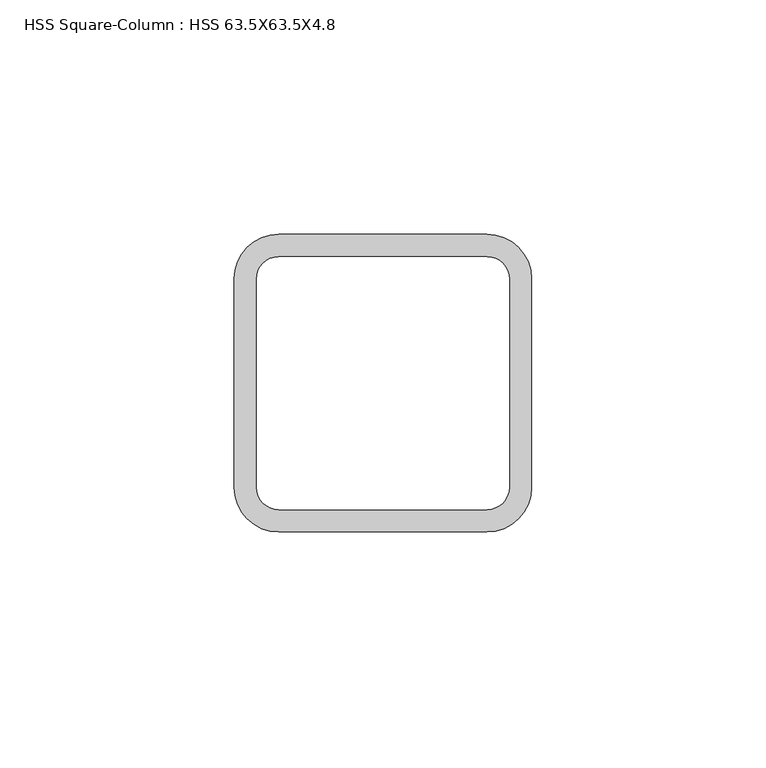
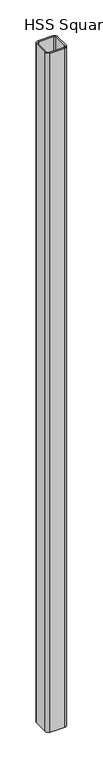
"""IFC4 building model written with IfcOpenShell, lengths in millimetres: column geometry, HSS Square-Column : HSS 63.5X63.5X4.8."""

from ifc_helpers import new_model, si_unit, point, frame, frame_2d, origin, place, context, project, spatial, polyline, circle_curve, trimmed, segment, composite_curve, outline, extrude, source, transform, mapped, element, save


def hss_square_column_hss_63_5x63_5x4_8_a081246b(model_context):
    return source(origin(), model_context, "Body", "SweptSolid", [
        extrude(outline(composite_curve([segment(trimmed(circle_curve(frame_2d((22.225, 22.225)), 9.525), [point((22.225, 31.75))], [point((31.75, 22.225))], False, "CARTESIAN"), True, "CONTINUOUS"), segment(polyline([(31.75, 22.225), (31.75, -22.225)]), True, "CONTINUOUS"), segment(trimmed(circle_curve(frame_2d((22.225, -22.225)), 9.525), [point((31.75, -22.225))], [point((22.225, -31.75))], False, "CARTESIAN"), True, "CONTINUOUS"), segment(polyline([(22.225, -31.75), (-22.225, -31.75)]), True, "CONTINUOUS"), segment(trimmed(circle_curve(frame_2d((-22.225, -22.225)), 9.525), [point((-22.225, -31.75))], [point((-31.75, -22.225))], False, "CARTESIAN"), True, "CONTINUOUS"), segment(polyline([(-31.75, -22.225), (-31.75, 22.225)]), True, "CONTINUOUS"), segment(trimmed(circle_curve(frame_2d((-22.225, 22.225)), 9.525), [point((-31.75, 22.225))], [point((-22.225, 31.75))], False, "CARTESIAN"), True, "CONTINUOUS"), segment(polyline([(-22.225, 31.75), (22.225, 31.75)]), True, "CONTINUOUS")], self_intersect=False), holes=[composite_curve([segment(polyline([(22.225, 26.9875), (-22.225, 26.9875)]), True, "CONTINUOUS"), segment(trimmed(circle_curve(frame_2d((-22.225, 22.225)), 4.7625), [point((-22.225, 26.9875))], [point((-26.9875, 22.225))], True, "CARTESIAN"), True, "CONTINUOUS"), segment(polyline([(-26.9875, 22.225), (-26.9875, -22.225)]), True, "CONTINUOUS"), segment(trimmed(circle_curve(frame_2d((-22.225, -22.225)), 4.7625), [point((-26.9875, -22.225))], [point((-22.225, -26.9875))], True, "CARTESIAN"), True, "CONTINUOUS"), segment(polyline([(-22.225, -26.9875), (22.225, -26.9875)]), True, "CONTINUOUS"), segment(trimmed(circle_curve(frame_2d((22.225, -22.225)), 4.7625), [point((22.225, -26.9875))], [point((26.9875, -22.225))], True, "CARTESIAN"), True, "CONTINUOUS"), segment(polyline([(26.9875, -22.225), (26.9875, 22.225)]), True, "CONTINUOUS"), segment(trimmed(circle_curve(frame_2d((22.225, 22.225)), 4.7625), [point((26.9875, 22.225))], [point((22.225, 26.9875))], True, "CARTESIAN"), True, "CONTINUOUS")], self_intersect=False)]), frame((0.0, 0.0, 3220.0), z_axis=(0.0, 0.0, 1.0), x_axis=(1.0, 0.0, 0.0)), (0.0, 0.0, 1.0), 2150.0),
    ])


if __name__ == "__main__":
    model = new_model("IFC4")
    model_context = context("Model", 3, world=origin())
    ifc_project = project(units=[si_unit("LENGTHUNIT", "METRE", prefix="MILLI")], contexts=[model_context])
    site = spatial("IfcSite", under=ifc_project)
    building = spatial("IfcBuilding", under=site)
    placement = place(None, origin())
    hss_square_column_hss_63_5x63_5x4_8_shape = hss_square_column_hss_63_5x63_5x4_8_a081246b(model_context)
    element("IfcColumn", 1, ObjectType="HSS Square-Column : HSS 63.5X63.5X4.8", at=placement, inside=building, context=model_context, shape_type="MappedRepresentation", body=[
        mapped(hss_square_column_hss_63_5x63_5x4_8_shape, transform((0.0, 0.0, 0.0), x_axis=(1.0, 0.0, 0.0), y_axis=(0.0, 1.0, 0.0), z_axis=(0.0, 0.0, 1.0))),
    ])
    save(model, "model.ifc")

# Revit data of these elements
# Type "HSS Square-Column : HSS 63.5X63.5X4.8"
#   Section Name Key = "HSS 2 1/2X2 1/2X3/16"
#   Assembly Code = "B10"
#   Width = 6.35 cm
#   Wall Nominal Thickness = 0.4763 cm
#   Wall Design Thickness = 0.442 cm
#   Torsional Moment of Inertia = 93.6521 cm⁴
#   Torsional Modulus = 30.4799 cm³
#   Section Area = 9.93546 cm²
#   Plastic Modulus weak axis = 21.6309 cm³
#   Plastic Modulus strong axis = 21.6309 cm³
#   Outer Fillet = 0.9525 cm
#   Nominal Weight = 8.31884 kgf/m
#   Moment of Inertia weak axis = 56.1912 cm⁴
#   Moment of Inertia strong axis = 56.1912 cm⁴
#   Inner Fillet = 0.4763 cm
#   Height = 6.35 cm
#   Elastic Modulus weak axis = 17.698 cm³
#   Elastic Modulus strong axis = 17.698 cm³
#   Centroid Vertical = 3.175 cm
#   Centroid Horizontal = 3.175 cm
#   Structural Material [instance default] = Steel ASTM A500, Grade B, Rectangular and Square
#   Principal Axes Angle = 0
# Element 1 (IfcColumn, "HSS Square-Column : HSS 63.5X63.5X4.8")
#   Structural Material = none
# Materials
#   "Steel ASTM A500, Grade B, Rectangular and Square": class "Metal", colour RGB 199 199 199, transparency 0, Description = "Carbon steel", Cost = 0
